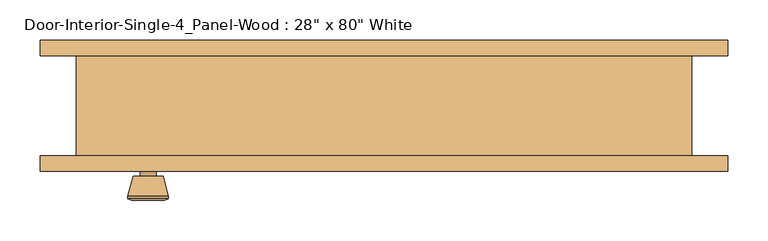
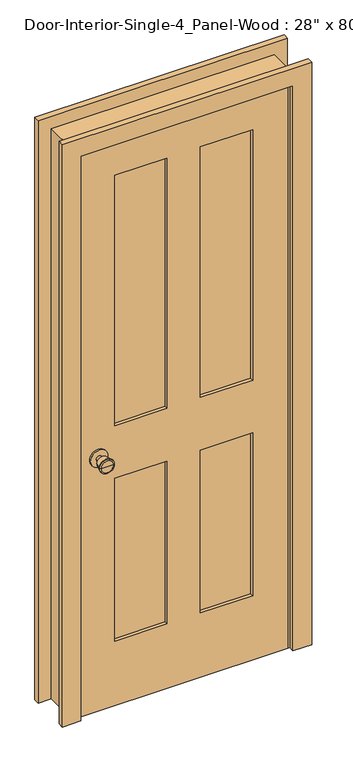
"""IFC4 building model written with IfcOpenShell, lengths in millimetres: door geometry."""

from ifc_helpers import new_model, si_unit, point, frame, frame_2d, origin, place, context, project, spatial, polyline, circle_curve, trimmed, segment, composite_curve, outline, extrude, faceted_brep, source, transform, mapped, element, save
from ifc_brep_helpers import plane_surface, cylinder_surface, revolved_surface, advanced_brep


def door_fc23bb36(model_context):
    return source(origin(), model_context, "Body", "SolidModel", [
        advanced_brep(
        [(-292.1, -17.8125, 914.4), (-302.1, -17.8125, 914.4), (-282.1, -17.8125, 914.4), (-271.6241324, 31.1875, 914.4), (-312.5758676, 31.1875, 914.4), (-292.1, 31.1875, 914.4), (-267.1, 29.3596319, 914.4), (-317.1, 29.3596319, 914.4), (-267.1, 25.8959537, 914.4), (-317.1, 25.8959537, 914.4), (-273.463764, 1.1875, 914.4), (-310.736236, 1.1875, 914.4), (-282.1, 1.1875, 914.4), (-302.1, 1.1875, 914.4)],
        [
            (0, 1),
            (1, 2, circle_curve(frame((-292.1, -17.8125, 914.4), z_axis=(0.0, -1.0, 0.0), x_axis=(-1.0, 0.0, 0.0)), 10.0)),
            (2, 0),
            (2, 1, circle_curve(frame((-292.1, -17.8125, 914.4), z_axis=(0.0, -1.0, 0.0), x_axis=(-1.0, 0.0, 0.0)), 10.0)),
            (3, 4, circle_curve(frame((-292.1, 31.1875, 914.4), z_axis=(0.0, 1.0, 0.0), x_axis=(-1.0, 0.0, 0.0)), 20.4758676)),
            (4, 5),
            (5, 3),
            (4, 3, circle_curve(frame((-292.1, 31.1875, 914.4), z_axis=(0.0, 1.0, 0.0), x_axis=(-1.0, 0.0, 0.0)), 20.4758676)),
            (6, 7, circle_curve(frame((-292.1, 29.3596319, 914.4), z_axis=(0.0, 1.0, 0.0), x_axis=(-1.0, 0.0, 0.0)), 25.0)),
            (7, 4),
            (3, 6),
            (7, 6, circle_curve(frame((-292.1, 29.3596319, 914.4), z_axis=(0.0, 1.0, 0.0), x_axis=(-1.0, 0.0, 0.0)), 25.0)),
            (8, 9, circle_curve(frame((-292.1, 25.8959537, 914.4), z_axis=(0.0, 1.0, 0.0), x_axis=(-1.0, 0.0, 0.0)), 25.0)),
            (9, 7),
            (6, 8),
            (9, 8, circle_curve(frame((-292.1, 25.8959537, 914.4), z_axis=(0.0, 1.0, 0.0), x_axis=(-1.0, 0.0, 0.0)), 25.0)),
            (10, 11, circle_curve(frame((-292.1, 1.1875, 914.4), z_axis=(0.0, 1.0, 0.0), x_axis=(-1.0, 0.0, 0.0)), 18.636236)),
            (11, 9),
            (8, 10),
            (11, 10, circle_curve(frame((-292.1, 1.1875, 914.4), z_axis=(0.0, 1.0, 0.0), x_axis=(-1.0, 0.0, 0.0)), 18.636236)),
            (12, 13, circle_curve(frame((-292.1, 1.1875, 914.4), z_axis=(0.0, 1.0, 0.0), x_axis=(-1.0, 0.0, 0.0)), 10.0)),
            (13, 11),
            (10, 12),
            (13, 12, circle_curve(frame((-292.1, 1.1875, 914.4), z_axis=(0.0, 1.0, 0.0), x_axis=(-1.0, 0.0, 0.0)), 10.0)),
            (1, 13),
            (12, 2),
        ],
        [
            plane_surface(frame((-292.1, -17.8125, 914.4), z_axis=(0.0, -1.0, 0.0), x_axis=(-1.0, 0.0, 0.0))),
            plane_surface(frame((-292.1, 31.1875, 914.4), z_axis=(0.0, 1.0, 0.0), x_axis=(-1.0, 0.0, 0.0))),
            revolved_surface(polyline([(-312.5758676, 31.1875, 914.4), (-317.1, 29.3596319, 914.4)]), (-292.1, -17.8125, 914.4), (0.0, -1.0, 0.0)),
            cylinder_surface(frame((-292.1, -17.8125, 914.4), z_axis=(0.0, -1.0, 0.0), x_axis=(-1.0, 0.0, 0.0)), 25.0),
            revolved_surface(polyline([(-317.1, 25.8959537, 914.4), (-310.736236, 1.1875, 914.4)]), (-292.1, -17.8125, 914.4), (0.0, -1.0, 0.0)),
            plane_surface(frame((-292.1, 1.1875, 914.4), z_axis=(0.0, -1.0, 0.0), x_axis=(-1.0, 0.0, 0.0))),
            cylinder_surface(frame((-292.1, -17.8125, 914.4), z_axis=(0.0, -1.0, 0.0), x_axis=(-1.0, 0.0, 0.0)), 10.0),
        ],
        [
            (0, [[1, 2, 3]]),
            (0, [[-3, 4, -1]]),
            (1, [[5, 6, 7]]),
            (1, [[8, -7, -6]]),
            (2, [[9, 10, -5, 11]]),
            (2, [[12, -11, -8, -10]]),
            (3, [[13, 14, -9, 15]]),
            (3, [[16, -15, -12, -14]]),
            (4, [[17, 18, -13, 19]]),
            (4, [[20, -19, -16, -18]]),
            (5, [[21, 22, -17, 23]]),
            (5, [[24, -23, -20, -22]]),
            (6, [[-2, 25, -21, 26]]),
            (6, [[-4, -26, -24, -25]]),
        ],
    ),
        extrude(outline(composite_curve([segment(trimmed(circle_curve(frame_2d((914.4, -292.1)), 30.0), [point((914.4, -322.1))], [point((914.4, -262.1))], False, "CARTESIAN"), True, "CONTINUOUS"), segment(trimmed(circle_curve(frame_2d((914.4, -292.1)), 30.0), [point((914.4, -262.1))], [point((914.4, -322.1))], False, "CARTESIAN"), True, "CONTINUOUS")], self_intersect=False)), frame((0.0, -23.8125, 0.0), z_axis=(0.0, 1.0, 0.0), x_axis=(0.0, 0.0, 1.0)), (0.0, 0.0, 1.0), 6.0),
        advanced_brep(
        [(-292.1, -64.7375, 914.4), (-282.1, -64.7375, 914.4), (-302.1, -64.7375, 914.4), (-271.6241324, -113.7375, 914.4), (-292.1, -113.7375, 914.4), (-312.5758676, -113.7375, 914.4), (-267.1, -111.9096319, 914.4), (-317.1, -111.9096319, 914.4), (-267.1, -108.4459537, 914.4), (-317.1, -108.4459537, 914.4), (-273.463764, -83.7375, 914.4), (-310.736236, -83.7375, 914.4), (-282.1, -83.7375, 914.4), (-302.1, -83.7375, 914.4)],
        [
            (0, 1),
            (1, 2, circle_curve(frame((-292.1, -64.7375, 914.4), z_axis=(0.0, 1.0, 0.0), x_axis=(-1.0, 0.0, 0.0)), 10.0)),
            (2, 0),
            (2, 1, circle_curve(frame((-292.1, -64.7375, 914.4), z_axis=(0.0, 1.0, 0.0), x_axis=(-1.0, 0.0, 0.0)), 10.0)),
            (3, 4),
            (4, 5),
            (5, 3, circle_curve(frame((-292.1, -113.7375, 914.4), z_axis=(0.0, -1.0, 0.0), x_axis=(-1.0, 0.0, 0.0)), 20.4758676)),
            (3, 5, circle_curve(frame((-292.1, -113.7375, 914.4), z_axis=(0.0, -1.0, 0.0), x_axis=(-1.0, 0.0, 0.0)), 20.4758676)),
            (6, 3),
            (5, 7),
            (7, 6, circle_curve(frame((-292.1, -111.9096319, 914.4), z_axis=(0.0, -1.0, 0.0), x_axis=(-1.0, 0.0, 0.0)), 25.0)),
            (6, 7, circle_curve(frame((-292.1, -111.9096319, 914.4), z_axis=(0.0, -1.0, 0.0), x_axis=(-1.0, 0.0, 0.0)), 25.0)),
            (8, 6),
            (7, 9),
            (9, 8, circle_curve(frame((-292.1, -108.4459537, 914.4), z_axis=(0.0, -1.0, 0.0), x_axis=(-1.0, 0.0, 0.0)), 25.0)),
            (8, 9, circle_curve(frame((-292.1, -108.4459537, 914.4), z_axis=(0.0, -1.0, 0.0), x_axis=(-1.0, 0.0, 0.0)), 25.0)),
            (10, 8),
            (9, 11),
            (11, 10, circle_curve(frame((-292.1, -83.7375, 914.4), z_axis=(0.0, -1.0, 0.0), x_axis=(-1.0, 0.0, 0.0)), 18.636236)),
            (10, 11, circle_curve(frame((-292.1, -83.7375, 914.4), z_axis=(0.0, -1.0, 0.0), x_axis=(-1.0, 0.0, 0.0)), 18.636236)),
            (12, 10),
            (11, 13),
            (13, 12, circle_curve(frame((-292.1, -83.7375, 914.4), z_axis=(0.0, -1.0, 0.0), x_axis=(-1.0, 0.0, 0.0)), 10.0)),
            (12, 13, circle_curve(frame((-292.1, -83.7375, 914.4), z_axis=(0.0, -1.0, 0.0), x_axis=(-1.0, 0.0, 0.0)), 10.0)),
            (1, 12),
            (13, 2),
        ],
        [
            plane_surface(frame((-292.1, -64.7375, 914.4), z_axis=(0.0, 1.0, 0.0), x_axis=(-1.0, 0.0, 0.0))),
            plane_surface(frame((-292.1, -113.7375, 914.4), z_axis=(0.0, -1.0, 0.0), x_axis=(-1.0, 0.0, 0.0))),
            revolved_surface(polyline([(-312.5758676, -113.7375, 914.4), (-317.1, -111.9096319, 914.4)]), (-292.1, -64.7375, 914.4), (0.0, 1.0, 0.0)),
            cylinder_surface(frame((-292.1, -64.7375, 914.4), z_axis=(0.0, 1.0, 0.0), x_axis=(-1.0, 0.0, 0.0)), 25.0),
            revolved_surface(polyline([(-317.1, -108.4459537, 914.4), (-310.736236, -83.7375, 914.4)]), (-292.1, -64.7375, 914.4), (0.0, 1.0, 0.0)),
            plane_surface(frame((-292.1, -83.7375, 914.4), z_axis=(0.0, 1.0, 0.0), x_axis=(-1.0, 0.0, 0.0))),
            cylinder_surface(frame((-292.1, -64.7375, 914.4), z_axis=(0.0, 1.0, 0.0), x_axis=(-1.0, 0.0, 0.0)), 10.0),
        ],
        [
            (0, [[1, 2, 3]]),
            (0, [[-3, 4, -1]]),
            (1, [[5, 6, 7]]),
            (1, [[-6, -5, 8]]),
            (2, [[9, -7, 10, 11]]),
            (2, [[-10, -8, -9, 12]]),
            (3, [[13, -11, 14, 15]]),
            (3, [[-14, -12, -13, 16]]),
            (4, [[17, -15, 18, 19]]),
            (4, [[-18, -16, -17, 20]]),
            (5, [[21, -19, 22, 23]]),
            (5, [[-22, -20, -21, 24]]),
            (6, [[25, -23, 26, -2]]),
            (6, [[-26, -24, -25, -4]]),
        ],
    ),
        extrude(outline(composite_curve([segment(trimmed(circle_curve(frame_2d((914.4, -292.1)), 30.0), [point((914.4, -322.1))], [point((914.4, -262.1))], False, "CARTESIAN"), True, "CONTINUOUS"), segment(trimmed(circle_curve(frame_2d((914.4, -292.1)), 30.0), [point((914.4, -262.1))], [point((914.4, -322.1))], False, "CARTESIAN"), True, "CONTINUOUS")], self_intersect=False)), frame((0.0, -64.7375, 0.0), z_axis=(0.0, 1.0, 0.0), x_axis=(0.0, 0.0, 1.0)), (0.0, 0.0, 1.0), 6.0),
        extrude(outline(polyline([(234.95, -35.4541667), (234.95, -47.0958333), (57.15, -47.0958333), (57.15, -35.4541667), (234.95, -35.4541667)])), frame((0.0, 0.0, 1009.65), z_axis=(0.0, 0.0, 1.0), x_axis=(1.0, 0.0, 0.0)), (0.0, 0.0, 1.0), 903.2875),
        extrude(outline(polyline([(-57.15, -35.4541667), (-57.15, -47.0958333), (-234.95, -47.0958333), (-234.95, -35.4541667), (-57.15, -35.4541667)])), frame((0.0, 0.0, 1009.65), z_axis=(0.0, 0.0, 1.0), x_axis=(1.0, 0.0, 0.0)), (0.0, 0.0, 1.0), 903.2875),
        extrude(outline(polyline([(234.95, -35.4541667), (234.95, -47.0958333), (57.15, -47.0958333), (57.15, -35.4541667), (234.95, -35.4541667)])), frame((0.0, 0.0, 231.775), z_axis=(0.0, 0.0, 1.0), x_axis=(1.0, 0.0, 0.0)), (0.0, 0.0, 1.0), 587.375),
        extrude(outline(polyline([(-57.15, -35.4541667), (-57.15, -47.0958333), (-234.95, -47.0958333), (-234.95, -35.4541667), (-57.15, -35.4541667)])), frame((0.0, 0.0, 231.775), z_axis=(0.0, 0.0, 1.0), x_axis=(1.0, 0.0, 0.0)), (0.0, 0.0, 1.0), 587.375),
        extrude(outline(polyline([(2032.0, -355.6), (0.0, -355.6), (0.0, 355.6), (2032.0, 355.6), (2032.0, -355.6)]), holes=[polyline([(1912.9375, 57.15), (1912.9375, 234.95), (1009.65, 234.95), (1009.65, 57.15), (1912.9375, 57.15)]), polyline([(1009.65, -57.15), (1009.65, -234.95), (1912.9375, -234.95), (1912.9375, -57.15), (1009.65, -57.15)]), polyline([(819.15, 57.15), (819.15, 234.95), (231.775, 234.95), (231.775, 57.15), (819.15, 57.15)]), polyline([(231.775, -57.15), (231.775, -234.95), (819.15, -234.95), (819.15, -57.15), (231.775, -57.15)])]), frame((0.0, -58.7375, 0.0), z_axis=(0.0, 1.0, 0.0), x_axis=(0.0, 0.0, 1.0)), (0.0, 0.0, 1.0), 34.925),
        faceted_brep([(381.0, -58.7375, 0.0), (355.6, -58.7375, 0.0), (355.6, -23.8125, 0.0), (342.9, -23.8125, 0.0), (342.9, 11.1125, 0.0), (355.6, 11.1125, 0.0), (355.6, 65.0875, 0.0), (381.0, 65.0875, 0.0), (381.0, 65.0875, 2057.4), (381.0, -58.7375, 2057.4), (355.6, 65.0875, 2032.0), (-355.6, 65.0875, 2032.0), (-355.6, 65.0875, 0.0), (-381.0, 65.0875, 0.0), (-381.0, 65.0875, 2057.4), (355.6, 11.1125, 2032.0), (342.9, 11.1125, 2019.3), (-342.9, 11.1125, 2019.3), (-342.9, 11.1125, 0.0), (-355.6, 11.1125, 0.0), (-355.6, 11.1125, 2032.0), (342.9, -23.8125, 2019.3), (355.6, -23.8125, 2032.0), (-355.6, -23.8125, 2032.0), (-355.6, -23.8125, 0.0), (-342.9, -23.8125, 0.0), (-342.9, -23.8125, 2019.3), (355.6, -58.7375, 2032.0), (-381.0, -58.7375, 2057.4), (-381.0, -58.7375, 0.0), (-355.6, -58.7375, 0.0), (-355.6, -58.7375, 2032.0)], [[[0, 1, 2, 3, 4, 5, 6, 7]], [[7, 8, 9, 0]], [[6, 10, 11, 12, 13, 14, 8, 7]], [[5, 15, 10, 6]], [[4, 16, 17, 18, 19, 20, 15, 5]], [[3, 21, 16, 4]], [[2, 22, 23, 24, 25, 26, 21, 3]], [[1, 27, 22, 2]], [[0, 9, 28, 29, 30, 31, 27, 1]], [[8, 14, 28, 9]], [[15, 20, 11, 10]], [[21, 26, 17, 16]], [[27, 31, 23, 22]], [[29, 13, 12, 19, 18, 25, 24, 30]], [[14, 13, 29, 28]], [[20, 19, 12, 11]], [[26, 25, 18, 17]], [[31, 30, 24, 23]]]),
        extrude(outline(polyline([(0.0, 425.45), (2101.85, 425.45), (2101.85, -425.45), (0.0, -425.45), (0.0, -361.95), (2038.35, -361.95), (2038.35, 361.95), (0.0, 361.95), (0.0, 425.45)])), frame((0.0, 65.0875, 0.0), z_axis=(0.0, 1.0, 0.0), x_axis=(0.0, 0.0, 1.0)), (0.0, 0.0, 1.0), 19.05),
        extrude(outline(polyline([(0.0, 425.45), (2101.85, 425.45), (2101.85, -425.45), (0.0, -425.45), (0.0, -361.95), (2038.35, -361.95), (2038.35, 361.95), (0.0, 361.95), (0.0, 425.45)])), frame((0.0, -77.7875, 0.0), z_axis=(0.0, 1.0, 0.0), x_axis=(0.0, 0.0, 1.0)), (0.0, 0.0, 1.0), 19.05),
    ])


if __name__ == "__main__":
    model = new_model("IFC4")
    model_context = context("Model", 3, world=origin())
    ifc_project = project(units=[si_unit("LENGTHUNIT", "METRE", prefix="MILLI")], contexts=[model_context])
    site = spatial("IfcSite", under=ifc_project)
    building = spatial("IfcBuilding", under=site)
    placement = place(None, origin())
    door_shape = door_fc23bb36(model_context)
    element("IfcDoor", 1, ObjectType="Door-Interior-Single-4_Panel-Wood : 28\" x 80\" White", at=placement, inside=building, context=model_context, shape_type="MappedRepresentation", body=[
        mapped(door_shape, transform((0.0, 0.0, 0.0), x_axis=(1.0, 0.0, 0.0), y_axis=(0.0, 1.0, 0.0), z_axis=(0.0, 0.0, 1.0))),
    ])
    save(model, "model.ifc")

# Revit data of these elements
# Type "Door-Interior-Single-4_Panel-Wood : 28\" x 80\" White"
#   Type Mark = "72"
#   COBie.Type.CreatedBy = "doug.wood@us.ibm.com"
#   COBie.Type.CreatedOn = "2016-04-14T02:07:24"
#   COBie.Type.Name = "Doors_Door-Interior-Single-4_Panel-Wood_28\" x 80\" White_72"
#   COBie.Type.Category = "23-30 10 00 : Doors"
#   COBie.Type.Description = "Door-Interior-Single-4_Panel-Wood_28\" x 80\" White"
#   COBie.Type.Manufacturer = ""
#   COBie.Type.ModelNumber = ""
#   Assembly Code = "C1020300"
#   Analytic Construction = "Wooden"
#   COBie.Type.ReplacementCost = 0
#   Top Rail = 0' - 4 11/16"
#   Thickness = 0' - 1 3/8"
#   Thermal Resistance (R) = 0.455703 (m²·K)/W
#   Swing Angle [instance default] = 90.00°
#   Stiles = 0' - 4 3/4"
#   Rough Width = 2' - 6"
#   Rough Height = 6' - 9"
#   Mullion = 0' - 4 1/2"
#   Lock Rail = 0' - 7 1/2"
#   Height = 6' - 8"
#   Width = 2' - 4"
#   Heat Transfer Coefficient (U) = 2.19465 W/(m²·K)
#   Bottom Rail = 0' - 9 1/8"
#   COBie.Type = no
#   Trim Material = Trim - White
#   Panel Material = Door - Panel - White
#   Frame Material = Door - Panel - White
#   Door Handle Material = ARCAT - Metal - Brass, Polished
#   Visual Light Transmittance = 0
#   Solar Heat Gain Coefficient = 0
#   Wall Closure = (empty or 0)
#   Function = (empty or 0)
# Element 1 (IfcDoor, "Door-Interior-Single-4_Panel-Wood : 28\" x 80\" White")
#   Materials on its faces: "Door - Panel - White", "ARCAT - Metal - Brass, Polished", "Trim - White"
# Materials
#   "Trim - White": class "Wood", colour RGB 255 255 255, transparency 0, Cost = 0
#   "Door - Panel - White": class "Wood", colour RGB 255 255 255, transparency 0, Cost = 0
#   "ARCAT - Metal - Brass, Polished": class "Unassigned", colour RGB 246 240 166, transparency 0, Keynote = "05050", Model = "Generic", Manufacturer = "Generic", Description = "Steel, Chrome Plated"
